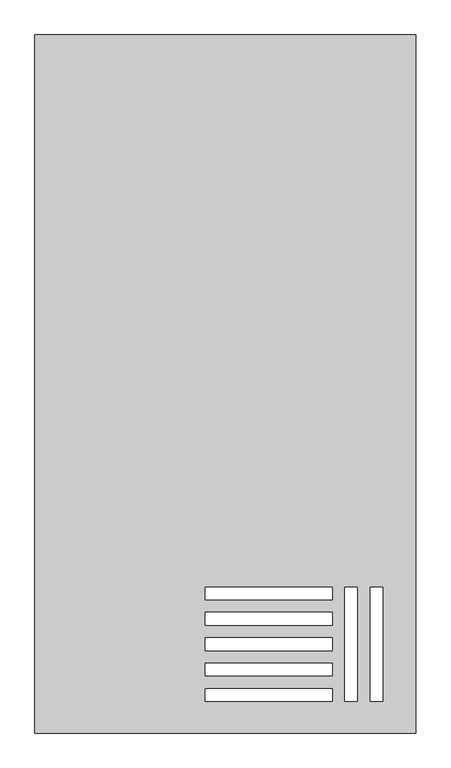
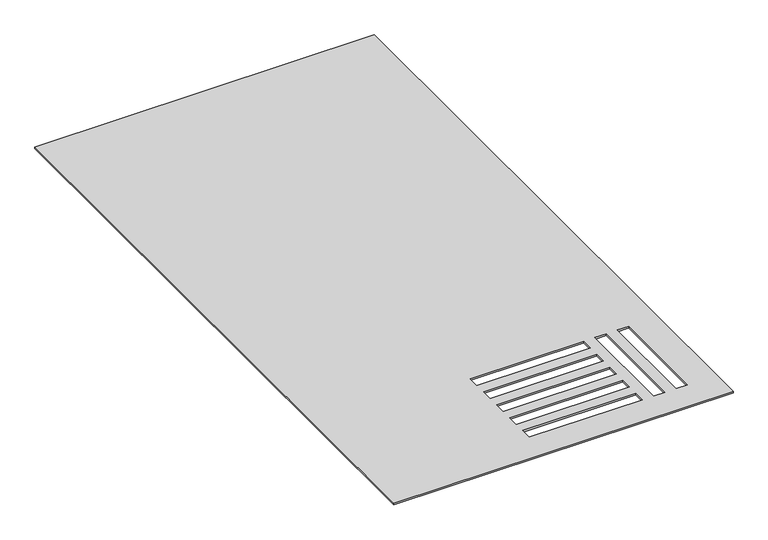
"""IFC4 building model written with IfcOpenShell, lengths in millimetres: proxy geometry, TSP Geyser Solar 250L : TSP Geyser Solar 250L."""

from ifc_helpers import new_model, si_unit, origin, origin_with_axes, place, context, project, spatial, polyline, outline, extrude, source, transform, mapped, element, save


def electrical_fixtures_e9d5f672(model_context):
    return source(origin(), model_context, "Body", "SweptSolid", [
        extrude(outline(polyline([(-600.0, 600.0), (0.0, 600.0), (0.0, -500.0), (-600.0, -500.0), (-600.0, 600.0)]), holes=[polyline([(-71.8082825, -450.0), (-51.8082825, -450.0), (-51.8082825, -270.0), (-71.8082825, -270.0), (-71.8082825, -450.0)]), polyline([(-131.8082825, -270.0), (-331.8082825, -270.0), (-331.8082825, -290.0), (-131.8082825, -290.0), (-131.8082825, -270.0)]), polyline([(-131.8082825, -310.0), (-331.8082825, -310.0), (-331.8082825, -330.0), (-131.8082825, -330.0), (-131.8082825, -310.0)]), polyline([(-131.8082825, -350.0), (-331.8082825, -350.0), (-331.8082825, -370.0), (-131.8082825, -370.0), (-131.8082825, -350.0)]), polyline([(-131.8082825, -390.0), (-331.8082825, -390.0), (-331.8082825, -410.0), (-131.8082825, -410.0), (-131.8082825, -390.0)]), polyline([(-131.8082825, -430.0), (-331.8082825, -430.0), (-331.8082825, -450.0), (-131.8082825, -450.0), (-131.8082825, -430.0)]), polyline([(-111.8082825, -450.0), (-91.8082825, -450.0), (-91.8082825, -270.0), (-111.8082825, -270.0), (-111.8082825, -450.0)])]), origin_with_axes(), (0.0, 0.0, 1.0), 3.0),
    ])


if __name__ == "__main__":
    model = new_model("IFC4")
    model_context = context("Model", 3, world=origin())
    ifc_project = project(units=[si_unit("LENGTHUNIT", "METRE", prefix="MILLI")], contexts=[model_context])
    site = spatial("IfcSite", under=ifc_project)
    building = spatial("IfcBuilding", under=site)
    placement = place(None, origin())
    electrical_fixtures_shape = electrical_fixtures_e9d5f672(model_context)
    element("IfcBuildingElementProxy", 1, Name="TSP Geyser Solar 250L : TSP Geyser Solar 250L", ObjectType="TSP Geyser Solar 250L : TSP Geyser Solar 250L", at=placement, inside=building, context=model_context, shape_type="MappedRepresentation", body=[
        mapped(electrical_fixtures_shape, transform((0.0, 0.0, 0.0), x_axis=(1.0, 0.0, 0.0), y_axis=(0.0, 1.0, 0.0), z_axis=(0.0, 0.0, 1.0))),
    ])
    save(model, "model.ifc")

# Revit data of these elements
# Type "TSP Geyser Solar 250L : TSP Geyser Solar 250L"
#   Model = "TSP_SGEY250"
#   Default Elevation = 0
# Element 1 (IfcBuildingElementProxy, "TSP Geyser Solar 250L : TSP Geyser Solar 250L")
#   Materials on its faces: "Aluminum, Anodized Red"
# Materials
#   "Aluminum, Anodized Red": class "Metal", colour RGB 120 120 120, transparency 0, Description = "Anodized aluminum, red", Cost = 0
